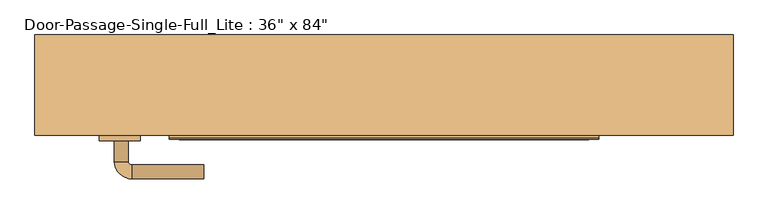
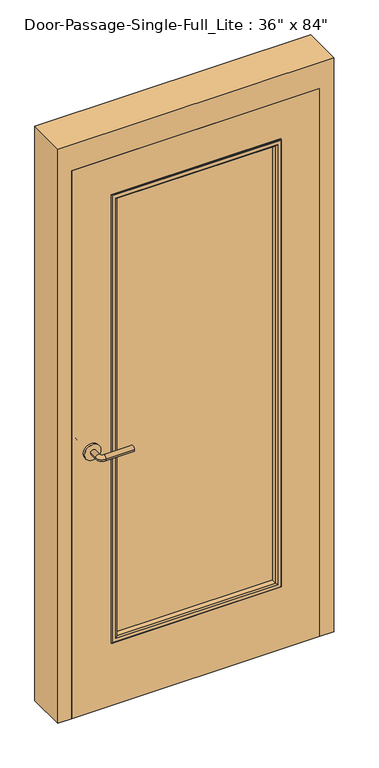
"""IFC4 building model written with IfcOpenShell, lengths in millimetres: door geometry."""

from ifc_helpers import new_model, si_unit, point, frame, frame_2d, origin, place, context, project, spatial, polyline, circle_curve, ellipse_curve, trimmed, segment, composite_curve, outline, extrude, faceted_brep, source, transform, mapped, element, save
from ifc_brep_helpers import plane_surface, cylinder_surface, revolved_surface, advanced_brep


def door_b5f71497(model_context):
    return source(origin(), model_context, "Body", "SolidModel", [
        advanced_brep(
        [(-392.190625, -15.8125, 1016.0), (-372.190625, -15.8125, 1016.0), (-392.190625, 14.1875, 1016.0), (-372.190625, 14.1875, 1016.0), (-367.190625, 19.1875, 1016.0), (-367.190625, 39.1875, 1016.0), (-262.190625, 39.1875, 1016.0), (-262.190625, 19.1875, 1016.0)],
        [
            (0, 1, circle_curve(frame((-382.190625, -15.8125, 1016.0), z_axis=(0.0, -1.0, 0.0), x_axis=(1.0, 0.0, 0.0)), 10.0)),
            (1, 0, circle_curve(frame((-382.190625, -15.8125, 1016.0), z_axis=(0.0, -1.0, 0.0), x_axis=(1.0, 0.0, 0.0)), 10.0)),
            (0, 2),
            (2, 3, circle_curve(frame((-382.190625, 14.1875, 1016.0), z_axis=(0.0, -1.0, 0.0), x_axis=(1.0, 0.0, 0.0)), 10.0)),
            (3, 1),
            (3, 2, circle_curve(frame((-382.190625, 14.1875, 1016.0), z_axis=(0.0, -1.0, 0.0), x_axis=(1.0, 0.0, 0.0)), 10.0)),
            (4, 3, circle_curve(frame((-367.190625, 14.1875, 1016.0), z_axis=(0.0, 0.0, 1.0), x_axis=(-1.0, 0.0, 0.0)), 5.0)),
            (2, 5, circle_curve(frame((-367.190625, 14.1875, 1016.0), z_axis=(0.0, 0.0, -1.0), x_axis=(-1.0, 0.0, 0.0)), 25.0)),
            (5, 4, circle_curve(frame((-367.190625, 29.1875, 1016.0), z_axis=(-1.0, 0.0, 0.0), x_axis=(0.0, -1.0, 0.0)), 10.0)),
            (4, 5, circle_curve(frame((-367.190625, 29.1875, 1016.0), z_axis=(-1.0, 0.0, 0.0), x_axis=(0.0, -1.0, 0.0)), 10.0)),
            (6, 7, circle_curve(frame((-262.190625, 29.1875, 1016.0), z_axis=(1.0, 0.0, 0.0), x_axis=(0.0, -1.0, 0.0)), 10.0)),
            (7, 6, circle_curve(frame((-262.190625, 29.1875, 1016.0), z_axis=(1.0, 0.0, 0.0), x_axis=(0.0, -1.0, 0.0)), 10.0)),
            (5, 6),
            (7, 4),
        ],
        [
            plane_surface(frame((-382.190625, -15.8125, 1016.0), z_axis=(0.0, -1.0, 0.0), x_axis=(0.0, 0.0, 1.0))),
            cylinder_surface(frame((-382.190625, -15.8125, 1016.0), z_axis=(0.0, -1.0, 0.0), x_axis=(1.0, 0.0, 0.0)), 10.0),
            revolved_surface(trimmed(ellipse_curve(frame((-382.190625, 14.1875, 1016.0), z_axis=(0.0, -1.0, 0.0), x_axis=(1.0, 0.0, 0.0)), 10.0, 10.0), [point((-392.190625, 14.1875, 1016.0))], [point((-372.190625, 14.1875, 1016.0))], True, "CARTESIAN"), (-367.190625, 14.1875, 1016.0), (0.0, 0.0, -1.0)),
            revolved_surface(trimmed(ellipse_curve(frame((-382.190625, 14.1875, 1016.0), z_axis=(0.0, -1.0, 0.0), x_axis=(1.0, 0.0, 0.0)), 10.0, 10.0), [point((-372.190625, 14.1875, 1016.0))], [point((-392.190625, 14.1875, 1016.0))], True, "CARTESIAN"), (-367.190625, 14.1875, 1016.0), (0.0, 0.0, -1.0)),
            plane_surface(frame((-262.190625, 29.1875, 1016.0), z_axis=(1.0, 0.0, 0.0), x_axis=(0.0, 0.0, 1.0))),
            cylinder_surface(frame((-367.190625, 29.1875, 1016.0), z_axis=(-1.0, 0.0, 0.0), x_axis=(0.0, -1.0, 0.0)), 10.0),
        ],
        [
            (0, [[1, 2]]),
            (1, [[-1, 3, 4, 5]]),
            (1, [[-2, -5, 6, -3]]),
            (2, [[7, -4, 8, 9]]),
            (3, [[-8, -6, -7, 10]]),
            (4, [[11, 12]]),
            (5, [[-9, 13, -12, 14]]),
            (5, [[-10, -14, -11, -13]]),
        ],
    ),
        extrude(outline(composite_curve([segment(trimmed(circle_curve(frame_2d((1016.0, -384.690625)), 30.0), [point((1016.0, -414.690625))], [point((1016.0, -354.690625))], False, "CARTESIAN"), True, "CONTINUOUS"), segment(trimmed(circle_curve(frame_2d((1016.0, -384.690625)), 30.0), [point((1016.0, -354.690625))], [point((1016.0, -414.690625))], False, "CARTESIAN"), True, "CONTINUOUS")], self_intersect=False)), frame((0.0, -23.8125, 0.0), z_axis=(0.0, 1.0, 0.0), x_axis=(0.0, 0.0, 1.0)), (0.0, 0.0, 1.0), 8.0),
        advanced_brep(
        [(-392.190625, -76.2625, 1016.0), (-372.190625, -76.2625, 1016.0), (-372.190625, -106.2625, 1016.0), (-392.190625, -106.2625, 1016.0), (-367.190625, -111.2625, 1016.0), (-367.190625, -131.2625, 1016.0), (-262.190625, -131.2625, 1016.0), (-262.190625, -111.2625, 1016.0)],
        [
            (0, 1, circle_curve(frame((-382.190625, -76.2625, 1016.0), z_axis=(0.0, 1.0, 0.0), x_axis=(1.0, 0.0, 0.0)), 10.0)),
            (1, 0, circle_curve(frame((-382.190625, -76.2625, 1016.0), z_axis=(0.0, 1.0, 0.0), x_axis=(1.0, 0.0, 0.0)), 10.0)),
            (1, 2),
            (2, 3, circle_curve(frame((-382.190625, -106.2625, 1016.0), z_axis=(0.0, 1.0, 0.0), x_axis=(1.0, 0.0, 0.0)), 10.0)),
            (3, 0),
            (3, 2, circle_curve(frame((-382.190625, -106.2625, 1016.0), z_axis=(0.0, 1.0, 0.0), x_axis=(1.0, 0.0, 0.0)), 10.0)),
            (4, 5, circle_curve(frame((-367.190625, -121.2625, 1016.0), z_axis=(-1.0, 0.0, 0.0), x_axis=(0.0, 1.0, 0.0)), 10.0)),
            (5, 3, circle_curve(frame((-367.190625, -106.2625, 1016.0), z_axis=(0.0, 0.0, -1.0), x_axis=(-1.0, 0.0, 0.0)), 25.0)),
            (2, 4, circle_curve(frame((-367.190625, -106.2625, 1016.0), z_axis=(0.0, 0.0, 1.0), x_axis=(-1.0, 0.0, 0.0)), 5.0)),
            (5, 4, circle_curve(frame((-367.190625, -121.2625, 1016.0), z_axis=(-1.0, 0.0, 0.0), x_axis=(0.0, 1.0, 0.0)), 10.0)),
            (6, 7, circle_curve(frame((-262.190625, -121.2625, 1016.0), z_axis=(1.0, 0.0, 0.0), x_axis=(0.0, 1.0, 0.0)), 10.0)),
            (7, 6, circle_curve(frame((-262.190625, -121.2625, 1016.0), z_axis=(1.0, 0.0, 0.0), x_axis=(0.0, 1.0, 0.0)), 10.0)),
            (4, 7),
            (6, 5),
        ],
        [
            plane_surface(frame((-382.190625, -76.2625, 1016.0), z_axis=(0.0, 1.0, 0.0), x_axis=(0.0, 0.0, 1.0))),
            cylinder_surface(frame((-382.190625, -76.2625, 1016.0), z_axis=(0.0, 1.0, 0.0), x_axis=(1.0, 0.0, 0.0)), 10.0),
            revolved_surface(trimmed(ellipse_curve(frame((-382.190625, -106.2625, 1016.0), z_axis=(0.0, -1.0, 0.0), x_axis=(1.0, 0.0, 0.0)), 10.0, 10.0), [point((-392.190625, -106.2625, 1016.0))], [point((-372.190625, -106.2625, 1016.0))], True, "CARTESIAN"), (-367.190625, -106.2625, 1016.0), (0.0, 0.0, -1.0)),
            revolved_surface(trimmed(ellipse_curve(frame((-382.190625, -106.2625, 1016.0), z_axis=(0.0, -1.0, 0.0), x_axis=(1.0, 0.0, 0.0)), 10.0, 10.0), [point((-372.190625, -106.2625, 1016.0))], [point((-392.190625, -106.2625, 1016.0))], True, "CARTESIAN"), (-367.190625, -106.2625, 1016.0), (0.0, 0.0, -1.0)),
            plane_surface(frame((-262.190625, -121.2625, 1016.0), z_axis=(1.0, 0.0, 0.0), x_axis=(0.0, 0.0, 1.0))),
            cylinder_surface(frame((-367.190625, -121.2625, 1016.0), z_axis=(-1.0, 0.0, 0.0), x_axis=(0.0, 1.0, 0.0)), 10.0),
        ],
        [
            (0, [[1, 2]]),
            (1, [[3, 4, 5, -2]]),
            (1, [[-5, 6, -3, -1]]),
            (2, [[7, 8, -4, 9]]),
            (3, [[10, -9, -6, -8]]),
            (4, [[11, 12]]),
            (5, [[13, -11, 14, -7]]),
            (5, [[-14, -12, -13, -10]]),
        ],
    ),
        extrude(outline(composite_curve([segment(trimmed(circle_curve(frame_2d((1016.0, -384.690625)), 30.0), [point((1016.0, -414.690625))], [point((1016.0, -354.690625))], False, "CARTESIAN"), True, "CONTINUOUS"), segment(trimmed(circle_curve(frame_2d((1016.0, -384.690625)), 30.0), [point((1016.0, -354.690625))], [point((1016.0, -414.690625))], False, "CARTESIAN"), True, "CONTINUOUS")], self_intersect=False)), frame((0.0, -76.2625, 0.0), z_axis=(0.0, 1.0, 0.0), x_axis=(0.0, 0.0, 1.0)), (0.0, 0.0, 1.0), 8.0),
        extrude(outline(polyline([(304.8, -42.8625), (304.8, -49.2125), (-304.8, -49.2125), (-304.8, -42.8625), (304.8, -42.8625)])), frame((0.0, 0.0, 254.0), z_axis=(0.0, 0.0, 1.0), x_axis=(1.0, 0.0, 0.0)), (0.0, 0.0, 1.0), 1727.2),
        faceted_brep([(457.2, -19.05, 0.0), (441.325, -19.05, 0.0), (441.325, 28.575, 0.0), (457.2, 28.575, 0.0), (457.2, 77.7875, 0.0), (508.0, 77.7875, 0.0), (508.0, -68.2625, 0.0), (457.2, -68.2625, 0.0), (457.2, -68.2625, 2133.6), (457.2, -19.05, 2133.6), (508.0, -68.2625, 2235.2), (-508.0, -68.2625, 2235.2), (-508.0, -68.2625, 0.0), (-457.2, -68.2625, 0.0), (-457.2, -68.2625, 2133.6), (508.0, 77.7875, 2235.2), (457.2, 77.7875, 2133.6), (-457.2, 77.7875, 2133.6), (-457.2, 77.7875, 0.0), (-508.0, 77.7875, 0.0), (-508.0, 77.7875, 2235.2), (457.2, 28.575, 2133.6), (441.325, 28.575, 2117.725), (-441.325, 28.575, 2117.725), (-441.325, 28.575, 0.0), (-457.2, 28.575, 0.0), (-457.2, 28.575, 2133.6), (441.325, -19.05, 2117.725), (-457.2, -19.05, 2133.6), (-457.2, -19.05, 0.0), (-441.325, -19.05, 0.0), (-441.325, -19.05, 2117.725)], [[[0, 1, 2, 3, 4, 5, 6, 7]], [[7, 8, 9, 0]], [[6, 10, 11, 12, 13, 14, 8, 7]], [[5, 15, 10, 6]], [[4, 16, 17, 18, 19, 20, 15, 5]], [[3, 21, 16, 4]], [[2, 22, 23, 24, 25, 26, 21, 3]], [[1, 27, 22, 2]], [[0, 9, 28, 29, 30, 31, 27, 1]], [[8, 14, 28, 9]], [[16, 21, 26, 17]], [[22, 27, 31, 23]], [[12, 19, 18, 25, 24, 30, 29, 13]], [[13, 29, 28, 14]], [[11, 20, 19, 12]], [[17, 26, 25, 18]], [[23, 31, 30, 24]], [[15, 20, 11, 10]]]),
        extrude(outline(polyline([(2133.6, -457.2), (0.0, -457.2), (0.0, 457.2), (2133.6, 457.2), (2133.6, -457.2)]), holes=[polyline([(1981.2, -304.8), (1981.2, 304.8), (254.0, 304.8), (254.0, -304.8), (1981.2, -304.8)])]), frame((0.0, -68.2625, 0.0), z_axis=(0.0, 1.0, 0.0), x_axis=(0.0, 0.0, 1.0)), (0.0, 0.0, 1.0), 44.45),
        advanced_brep(
        [(-304.8, -49.2125, 1981.2), (-304.8, -49.2125, 254.0), (-304.8, -68.2625, 254.0), (-304.8, -68.2625, 1981.2), (-292.8, -69.2625, 1969.2), (-292.8, -69.2625, 266.0), (-292.8, -49.2125, 266.0), (-292.8, -49.2125, 1969.2), (-297.8, -74.2625, 1974.2), (-297.8, -74.2625, 261.0), (-312.8, -72.2625, 1989.2), (-312.8, -72.2625, 246.0), (-310.8, -74.2625, 248.0), (-310.8, -74.2625, 1987.2), (-312.8, -68.2625, 1989.2), (-312.8, -68.2625, 246.0), (304.8, -49.2125, 254.0), (304.8, -68.2625, 254.0), (292.8, -69.2625, 266.0), (292.8, -49.2125, 266.0), (297.8, -74.2625, 261.0), (312.8, -72.2625, 246.0), (310.8, -74.2625, 248.0), (312.8, -68.2625, 246.0), (304.8, -49.2125, 1981.2), (304.8, -68.2625, 1981.2), (292.8, -69.2625, 1969.2), (292.8, -49.2125, 1969.2), (297.8, -74.2625, 1974.2), (312.8, -72.2625, 1989.2), (310.8, -74.2625, 1987.2), (312.8, -68.2625, 1989.2)],
        [
            (0, 1),
            (1, 2),
            (2, 3),
            (3, 0),
            (4, 5),
            (5, 6),
            (6, 7),
            (7, 4),
            (8, 9),
            (9, 5, ellipse_curve(frame((-297.8, -69.2625, 261.0), z_axis=(-0.7071067811865475, 0.0, 0.7071067811865475), x_axis=(0.7071067811865474, 0.0, 0.7071067811865476)), 7.0710678, 5.0)),
            (4, 8, ellipse_curve(frame((-297.8, -69.2625, 1974.2), z_axis=(-0.7071067811865475, 0.0, -0.7071067811865475), x_axis=(-0.7071067811865474, 0.0, 0.7071067811865476)), 7.0710678, 5.0)),
            (10, 11),
            (11, 12, ellipse_curve(frame((-310.8, -72.2625, 248.0), z_axis=(-0.7071067811865475, 0.0, 0.7071067811865475), x_axis=(0.7071067811865474, 0.0, 0.7071067811865476)), 2.8284271, 2.0)),
            (12, 13),
            (13, 10, ellipse_curve(frame((-310.8, -72.2625, 1987.2), z_axis=(-0.7071067811865475, 0.0, -0.7071067811865475), x_axis=(-0.7071067811865474, 0.0, 0.7071067811865476)), 2.8284271, 2.0)),
            (14, 15),
            (15, 11),
            (10, 14),
            (1, 16),
            (16, 17),
            (17, 2),
            (5, 18),
            (18, 19),
            (19, 6),
            (9, 20),
            (20, 18, ellipse_curve(frame((297.8, -69.2625, 261.0), z_axis=(-0.7071067811865475, 0.0, -0.7071067811865475), x_axis=(-0.7071067811865476, 0.0, 0.7071067811865474)), 7.0710678, 5.0)),
            (11, 21),
            (21, 22, ellipse_curve(frame((310.8, -72.2625, 248.0), z_axis=(-0.7071067811865475, 0.0, -0.7071067811865475), x_axis=(-0.7071067811865476, 0.0, 0.7071067811865474)), 2.8284271, 2.0)),
            (22, 12),
            (15, 23),
            (23, 21),
            (16, 24),
            (24, 25),
            (25, 17),
            (18, 26),
            (26, 27),
            (27, 19),
            (20, 28),
            (28, 26, ellipse_curve(frame((297.8, -69.2625, 1974.2), z_axis=(0.7071067811865475, 0.0, -0.7071067811865475), x_axis=(-0.7071067811865474, 0.0, -0.7071067811865476)), 7.0710678, 5.0)),
            (21, 29),
            (29, 30, ellipse_curve(frame((310.8, -72.2625, 1987.2), z_axis=(0.7071067811865475, 0.0, -0.7071067811865475), x_axis=(-0.7071067811865474, 0.0, -0.7071067811865476)), 2.8284271, 2.0)),
            (30, 22),
            (23, 31),
            (31, 29),
            (14, 31),
            (25, 3),
            (24, 0),
            (27, 7),
            (26, 4),
            (28, 8),
            (30, 13),
            (29, 10),
        ],
        [
            plane_surface(frame((-304.8, -68.2625, 1981.2), z_axis=(-1.0, 0.0, 0.0), x_axis=(0.0, 0.0, -1.0))),
            plane_surface(frame((-292.8, -49.2125, 1969.2), z_axis=(1.0, 0.0, 0.0), x_axis=(0.0, 0.0, -1.0))),
            cylinder_surface(frame((-297.8, -69.2625, 1981.2), z_axis=(0.0, 0.0, 1.0), x_axis=(-1.0, 0.0, 0.0)), 5.0),
            cylinder_surface(frame((-310.8, -72.2625, 1981.2), z_axis=(0.0, 0.0, 1.0), x_axis=(-1.0, 0.0, 0.0)), 2.0),
            plane_surface(frame((-312.8, -72.2625, 1989.2), z_axis=(-1.0, 0.0, 0.0), x_axis=(0.0, 0.0, -1.0))),
            plane_surface(frame((-304.8, -68.2625, 254.0), z_axis=(0.0, 0.0, -1.0), x_axis=(1.0, 0.0, 0.0))),
            plane_surface(frame((-292.8, -49.2125, 266.0), z_axis=(0.0, 0.0, 1.0), x_axis=(1.0, 0.0, 0.0))),
            cylinder_surface(frame((-304.8, -69.2625, 261.0), z_axis=(-1.0, 0.0, 0.0), x_axis=(0.0, 0.0, -1.0)), 5.0),
            cylinder_surface(frame((-304.8, -72.2625, 248.0), z_axis=(-1.0, 0.0, 0.0), x_axis=(0.0, 0.0, -1.0)), 2.0),
            plane_surface(frame((-312.8, -72.2625, 246.0), z_axis=(0.0, 0.0, -1.0), x_axis=(1.0, 0.0, 0.0))),
            plane_surface(frame((304.8, -68.2625, 254.0), z_axis=(1.0, 0.0, 0.0), x_axis=(0.0, 0.0, 1.0))),
            plane_surface(frame((292.8, -49.2125, 266.0), z_axis=(-1.0, 0.0, 0.0), x_axis=(0.0, 0.0, 1.0))),
            cylinder_surface(frame((297.8, -69.2625, 254.0), z_axis=(0.0, 0.0, -1.0), x_axis=(1.0, 0.0, 0.0)), 5.0),
            cylinder_surface(frame((310.8, -72.2625, 254.0), z_axis=(0.0, 0.0, -1.0), x_axis=(1.0, 0.0, 0.0)), 2.0),
            plane_surface(frame((312.8, -72.2625, 246.0), z_axis=(1.0, 0.0, 0.0), x_axis=(0.0, 0.0, 1.0))),
            plane_surface(frame((312.8, -68.2625, 1989.2), z_axis=(0.0, 1.0, 0.0), x_axis=(-1.0, 0.0, 0.0))),
            plane_surface(frame((304.8, -68.2625, 1981.2), z_axis=(0.0, 0.0, 1.0), x_axis=(-1.0, 0.0, 0.0))),
            plane_surface(frame((304.8, -49.2125, 1981.2), z_axis=(0.0, 1.0, 0.0), x_axis=(-1.0, 0.0, 0.0))),
            plane_surface(frame((292.8, -49.2125, 1969.2), z_axis=(0.0, 0.0, -1.0), x_axis=(-1.0, 0.0, 0.0))),
            cylinder_surface(frame((304.8, -69.2625, 1974.2), z_axis=(1.0, 0.0, 0.0), x_axis=(0.0, 0.0, 1.0)), 5.0),
            plane_surface(frame((297.8, -74.2625, 1974.2), z_axis=(0.0, -1.0, 0.0), x_axis=(-1.0, 0.0, 0.0))),
            cylinder_surface(frame((304.8, -72.2625, 1987.2), z_axis=(1.0, 0.0, 0.0), x_axis=(0.0, 0.0, 1.0)), 2.0),
            plane_surface(frame((312.8, -72.2625, 1989.2), z_axis=(0.0, 0.0, 1.0), x_axis=(-1.0, 0.0, 0.0))),
        ],
        [
            (0, [[1, 2, 3, 4]]),
            (1, [[5, 6, 7, 8]]),
            (2, [[9, 10, -5, 11]]),
            (3, [[12, 13, 14, 15]]),
            (4, [[16, 17, -12, 18]]),
            (5, [[19, 20, 21, -2]]),
            (6, [[22, 23, 24, -6]]),
            (7, [[25, 26, -22, -10]]),
            (8, [[27, 28, 29, -13]]),
            (9, [[30, 31, -27, -17]]),
            (10, [[32, 33, 34, -20]]),
            (11, [[35, 36, 37, -23]]),
            (12, [[38, 39, -35, -26]]),
            (13, [[40, 41, 42, -28]]),
            (14, [[43, 44, -40, -31]]),
            (15, [[-16, 45, -43, -30], [-3, -21, -34, 46]]),
            (16, [[47, -4, -46, -33]]),
            (17, [[-1, -47, -32, -19], [-7, -24, -37, 48]]),
            (18, [[49, -8, -48, -36]]),
            (19, [[50, -11, -49, -39]]),
            (20, [[-14, -29, -42, 51], [-9, -50, -38, -25]]),
            (21, [[52, -15, -51, -41]]),
            (22, [[-45, -18, -52, -44]]),
        ],
    ),
        advanced_brep(
        [(-304.8, -42.8625, 254.0), (-304.8, -42.8625, 1981.2), (-304.8, -23.8125, 1981.2), (-304.8, -23.8125, 254.0), (-292.8, -22.8125, 266.0), (-292.8, -22.8125, 1969.2), (-292.8, -42.8625, 1969.2), (-292.8, -42.8625, 266.0), (-297.8, -17.8125, 261.0), (-297.8, -17.8125, 1974.2), (-312.8, -19.8125, 246.0), (-312.8, -19.8125, 1989.2), (-310.8, -17.8125, 1987.2), (-310.8, -17.8125, 248.0), (-312.8, -23.8125, 246.0), (-312.8, -23.8125, 1989.2), (304.8, -42.8625, 1981.2), (304.8, -23.8125, 1981.2), (292.8, -22.8125, 1969.2), (292.8, -42.8625, 1969.2), (297.8, -17.8125, 1974.2), (312.8, -19.8125, 1989.2), (310.8, -17.8125, 1987.2), (312.8, -23.8125, 1989.2), (304.8, -42.8625, 254.0), (304.8, -23.8125, 254.0), (292.8, -22.8125, 266.0), (292.8, -42.8625, 266.0), (297.8, -17.8125, 261.0), (312.8, -19.8125, 246.0), (310.8, -17.8125, 248.0), (312.8, -23.8125, 246.0)],
        [
            (0, 1),
            (1, 2),
            (2, 3),
            (3, 0),
            (4, 5),
            (5, 6),
            (6, 7),
            (7, 4),
            (8, 9),
            (9, 5, ellipse_curve(frame((-297.8, -22.8125, 1974.2), z_axis=(-0.7071067811865475, 0.0, -0.7071067811865475), x_axis=(0.7071067811865474, 0.0, -0.7071067811865476)), 7.0710678, 5.0)),
            (4, 8, ellipse_curve(frame((-297.8, -22.8125, 261.0), z_axis=(-0.7071067811865475, 0.0, 0.7071067811865475), x_axis=(-0.7071067811865474, 0.0, -0.7071067811865476)), 7.0710678, 5.0)),
            (10, 11),
            (11, 12, ellipse_curve(frame((-310.8, -19.8125, 1987.2), z_axis=(-0.7071067811865475, 0.0, -0.7071067811865475), x_axis=(0.7071067811865474, 0.0, -0.7071067811865476)), 2.8284271, 2.0)),
            (12, 13),
            (13, 10, ellipse_curve(frame((-310.8, -19.8125, 248.0), z_axis=(-0.7071067811865475, 0.0, 0.7071067811865475), x_axis=(-0.7071067811865474, 0.0, -0.7071067811865476)), 2.8284271, 2.0)),
            (14, 15),
            (15, 11),
            (10, 14),
            (1, 16),
            (16, 17),
            (17, 2),
            (5, 18),
            (18, 19),
            (19, 6),
            (9, 20),
            (20, 18, ellipse_curve(frame((297.8, -22.8125, 1974.2), z_axis=(-0.7071067811865475, 0.0, 0.7071067811865475), x_axis=(-0.7071067811865476, 0.0, -0.7071067811865474)), 7.0710678, 5.0)),
            (11, 21),
            (21, 22, ellipse_curve(frame((310.8, -19.8125, 1987.2), z_axis=(-0.7071067811865475, 0.0, 0.7071067811865475), x_axis=(-0.7071067811865476, 0.0, -0.7071067811865474)), 2.8284271, 2.0)),
            (22, 12),
            (15, 23),
            (23, 21),
            (16, 24),
            (24, 25),
            (25, 17),
            (18, 26),
            (26, 27),
            (27, 19),
            (20, 28),
            (28, 26, ellipse_curve(frame((297.8, -22.8125, 261.0), z_axis=(0.7071067811865475, 0.0, 0.7071067811865475), x_axis=(-0.7071067811865474, 0.0, 0.7071067811865476)), 7.0710678, 5.0)),
            (21, 29),
            (29, 30, ellipse_curve(frame((310.8, -19.8125, 248.0), z_axis=(0.7071067811865475, 0.0, 0.7071067811865475), x_axis=(-0.7071067811865474, 0.0, 0.7071067811865476)), 2.8284271, 2.0)),
            (30, 22),
            (23, 31),
            (31, 29),
            (14, 31),
            (25, 3),
            (24, 0),
            (27, 7),
            (26, 4),
            (28, 8),
            (30, 13),
            (29, 10),
        ],
        [
            plane_surface(frame((-304.8, -23.8125, 254.0), z_axis=(-1.0, 0.0, 0.0), x_axis=(0.0, 0.0, 1.0))),
            plane_surface(frame((-292.8, -42.8625, 266.0), z_axis=(1.0, 0.0, 0.0), x_axis=(0.0, 0.0, 1.0))),
            cylinder_surface(frame((-297.8, -22.8125, 254.0), z_axis=(0.0, 0.0, -1.0), x_axis=(-1.0, 0.0, 0.0)), 5.0),
            cylinder_surface(frame((-310.8, -19.8125, 254.0), z_axis=(0.0, 0.0, -1.0), x_axis=(-1.0, 0.0, 0.0)), 2.0),
            plane_surface(frame((-312.8, -19.8125, 246.0), z_axis=(-1.0, 0.0, 0.0), x_axis=(0.0, 0.0, 1.0))),
            plane_surface(frame((-304.8, -23.8125, 1981.2), z_axis=(0.0, 0.0, 1.0), x_axis=(1.0, 0.0, 0.0))),
            plane_surface(frame((-292.8, -42.8625, 1969.2), z_axis=(0.0, 0.0, -1.0), x_axis=(1.0, 0.0, 0.0))),
            cylinder_surface(frame((-304.8, -22.8125, 1974.2), z_axis=(-1.0, 0.0, 0.0), x_axis=(0.0, 0.0, 1.0)), 5.0),
            cylinder_surface(frame((-304.8, -19.8125, 1987.2), z_axis=(-1.0, 0.0, 0.0), x_axis=(0.0, 0.0, 1.0)), 2.0),
            plane_surface(frame((-312.8, -19.8125, 1989.2), z_axis=(0.0, 0.0, 1.0), x_axis=(1.0, 0.0, 0.0))),
            plane_surface(frame((304.8, -23.8125, 1981.2), z_axis=(1.0, 0.0, 0.0), x_axis=(0.0, 0.0, -1.0))),
            plane_surface(frame((292.8, -42.8625, 1969.2), z_axis=(-1.0, 0.0, 0.0), x_axis=(0.0, 0.0, -1.0))),
            cylinder_surface(frame((297.8, -22.8125, 1981.2), z_axis=(0.0, 0.0, 1.0), x_axis=(1.0, 0.0, 0.0)), 5.0),
            cylinder_surface(frame((310.8, -19.8125, 1981.2), z_axis=(0.0, 0.0, 1.0), x_axis=(1.0, 0.0, 0.0)), 2.0),
            plane_surface(frame((312.8, -19.8125, 1989.2), z_axis=(1.0, 0.0, 0.0), x_axis=(0.0, 0.0, -1.0))),
            plane_surface(frame((312.8, -23.8125, 246.0), z_axis=(0.0, -1.0, 0.0), x_axis=(-1.0, 0.0, 0.0))),
            plane_surface(frame((304.8, -23.8125, 254.0), z_axis=(0.0, 0.0, -1.0), x_axis=(-1.0, 0.0, 0.0))),
            plane_surface(frame((304.8, -42.8625, 254.0), z_axis=(0.0, -1.0, 0.0), x_axis=(-1.0, 0.0, 0.0))),
            plane_surface(frame((292.8, -42.8625, 266.0), z_axis=(0.0, 0.0, 1.0), x_axis=(-1.0, 0.0, 0.0))),
            cylinder_surface(frame((304.8, -22.8125, 261.0), z_axis=(1.0, 0.0, 0.0), x_axis=(0.0, 0.0, -1.0)), 5.0),
            plane_surface(frame((297.8, -17.8125, 261.0), z_axis=(0.0, 1.0, 0.0), x_axis=(-1.0, 0.0, 0.0))),
            cylinder_surface(frame((304.8, -19.8125, 248.0), z_axis=(1.0, 0.0, 0.0), x_axis=(0.0, 0.0, -1.0)), 2.0),
            plane_surface(frame((312.8, -19.8125, 246.0), z_axis=(0.0, 0.0, -1.0), x_axis=(-1.0, 0.0, 0.0))),
        ],
        [
            (0, [[1, 2, 3, 4]]),
            (1, [[5, 6, 7, 8]]),
            (2, [[9, 10, -5, 11]]),
            (3, [[12, 13, 14, 15]]),
            (4, [[16, 17, -12, 18]]),
            (5, [[19, 20, 21, -2]]),
            (6, [[22, 23, 24, -6]]),
            (7, [[25, 26, -22, -10]]),
            (8, [[27, 28, 29, -13]]),
            (9, [[30, 31, -27, -17]]),
            (10, [[32, 33, 34, -20]]),
            (11, [[35, 36, 37, -23]]),
            (12, [[38, 39, -35, -26]]),
            (13, [[40, 41, 42, -28]]),
            (14, [[43, 44, -40, -31]]),
            (15, [[-16, 45, -43, -30], [-3, -21, -34, 46]]),
            (16, [[47, -4, -46, -33]]),
            (17, [[-1, -47, -32, -19], [-7, -24, -37, 48]]),
            (18, [[49, -8, -48, -36]]),
            (19, [[50, -11, -49, -39]]),
            (20, [[-14, -29, -42, 51], [-9, -50, -38, -25]]),
            (21, [[52, -15, -51, -41]]),
            (22, [[-45, -18, -52, -44]]),
        ],
    ),
    ])


if __name__ == "__main__":
    model = new_model("IFC4")
    model_context = context("Model", 3, world=origin())
    ifc_project = project(units=[si_unit("LENGTHUNIT", "METRE", prefix="MILLI")], contexts=[model_context])
    site = spatial("IfcSite", under=ifc_project)
    building = spatial("IfcBuilding", under=site)
    placement = place(None, origin())
    door_shape = door_b5f71497(model_context)
    element("IfcDoor", 1, ObjectType="Door-Passage-Single-Full_Lite : 36\" x 84\"", at=placement, inside=building, context=model_context, shape_type="MappedRepresentation", body=[
        mapped(door_shape, transform((0.0, 0.0, 0.0), x_axis=(1.0, 0.0, 0.0), y_axis=(0.0, 1.0, 0.0), z_axis=(0.0, 0.0, 1.0))),
    ])
    save(model, "model.ifc")

# Revit data of these elements
# Type "Door-Passage-Single-Full_Lite : 36\" x 84\""
#   Type Mark = "52"
#   Assembly Code = "B2030100"
#   Analytic Construction = "Wooden"
#   Thickness = 0' - 1 3/4"
#   Thermal Resistance (R) = 2.5876 (h·ft²·°F)/BTU
#   Swing Angle [instance default] = 90.00°
#   Strike Height = 3' - 4"
#   Rough Width [instance default] = 3' - 4"
#   Rough Height [instance default] = 7' - 4"
#   MF Opening Height [instance default] = 0' - 4"
#   MF Opening Width [instance default] = 0' - 4"
#   Inset Calculate [instance default] = 0' - 4"
#   Masonry Inset [instance default] = 0' - 1"
#   Height = 7' - 0"
#   Width = 3' - 0"
#   Heat Transfer Coefficient (U) = 0.3865 BTU/(h·ft²·°F)
#   Masonry Frame Depth = 0' - 5 3/4"
#   Masonry Frame [instance default] = yes
#   Function = 1
#   Dry Wall Frame [instance default] = no
#   Panel Material = Wood - Birch
#   Glazing = Glass
#   Glass Stop Material = Metal - Paint Finish - Grey
#   Frame Material = Metal - Paint Finish - Grey
#   Door Handle Material = Aluminum
#   Visual Light Transmittance = 0
#   Solar Heat Gain Coefficient = 0
#   Wall Closure = (empty or 0)
# Element 1 (IfcDoor, "Door-Passage-Single-Full_Lite : 36\" x 84\"")
#   Inset Calculate = 0' - 3"
#   Masonry Inset = 0' - 0"
#   Materials on its faces: "Metal - Paint Finish - Grey", "Aluminum", "Wood - Birch", "Glass"
# Materials
#   "Wood - Birch": class "Wood", colour RGB 166 116 52, transparency 0, Cost = 0
#   "Glass": class "Glass", colour RGB 0 128 192, transparency 0.75, Description = "Soda Lime Glass", Cost = 0
#   "Metal - Paint Finish - Grey": class "Paint", colour RGB 104 104 104, transparency 0, Cost = 0
#   "Aluminum": class "Metal", colour RGB 247 247 247, transparency 0, Description = "Aluminum 6061", Cost = 0
